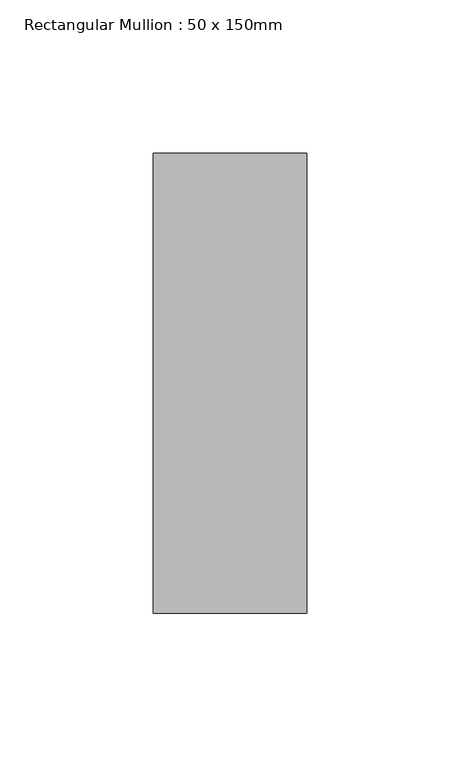
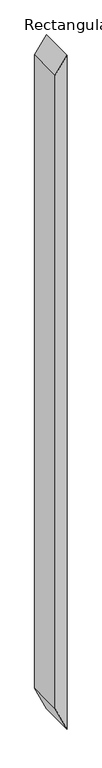
"""IFC4 building model written with IfcOpenShell, lengths in millimetres: member geometry, Rectangular Mullion : 50 x 150mm."""

from ifc_helpers import new_model, si_unit, frame, origin, place, context, project, spatial, polyline, outline, extrude, source, transform, mapped, element, save


def rectangular_mullion_50_x_150mm_a1351d1e(model_context):
    return source(origin(), model_context, "Body", "SweptSolid", [
        extrude(outline(polyline([(0.0, 0.0), (-71.6218739, -50.0), (-2906.9650483, -50.0), (-3015.6254931, 0.0), (0.0, 0.0)])), frame((0.0, -75.0, 0.0), z_axis=(0.0, 1.0, 0.0), x_axis=(0.0, 0.0, 1.0)), (0.0, 0.0, 1.0), 150.0),
    ])


if __name__ == "__main__":
    model = new_model("IFC4")
    model_context = context("Model", 3, world=origin())
    ifc_project = project(units=[si_unit("LENGTHUNIT", "METRE", prefix="MILLI")], contexts=[model_context])
    site = spatial("IfcSite", under=ifc_project)
    building = spatial("IfcBuilding", under=site)
    placement = place(None, origin())
    rectangular_mullion_50_x_150mm_shape = rectangular_mullion_50_x_150mm_a1351d1e(model_context)
    element("IfcMember", 1, ObjectType="Rectangular Mullion : 50 x 150mm", at=placement, inside=building, context=model_context, shape_type="MappedRepresentation", body=[
        mapped(rectangular_mullion_50_x_150mm_shape, transform((0.0, 0.0, 0.0), x_axis=(1.0, 0.0, 0.0), y_axis=(0.0, 1.0, 0.0), z_axis=(0.0, 0.0, 1.0))),
    ])
    save(model, "model.ifc")

# Revit data of these elements
# Type "Rectangular Mullion : 50 x 150mm"
#   built-in parameter 1007304 = 0.492126 (stored number, unit not read)
#   built-in parameter 1007301 = 0.082021 (stored number, unit not read)
#   built-in parameter 1007300 = 0.082021 (stored number, unit not read)
# Element 1 (IfcMember, "Rectangular Mullion : 50 x 150mm")
#   Materials on its faces: "Metal - Aluminium"
# Materials
#   "Metal - Aluminium": class "Metal", colour RGB 247 247 247, transparency 0
